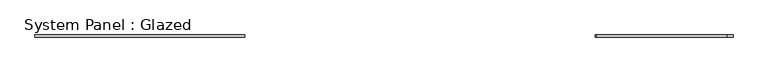
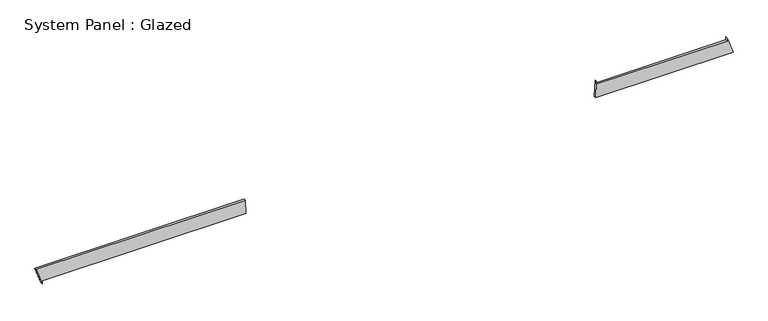
"""IFC4 building model written with IfcOpenShell, lengths in millimetres: plate geometry, System Panel : Glazed."""

from ifc_helpers import new_model, si_unit, frame, origin, place, context, project, spatial, polyline, outline, extrude, source, transform, mapped, element, save


def system_panel_glazed_a00b4466(model_context):
    return source(origin(), model_context, "Body", "SweptSolid", [
        extrude(outline(polyline([(0.0, -3957.6016429), (35.3553391, -3957.6016429), (35.3553391, -1604.6616071), (199.1260346, -1608.2248141), (199.0835123, -4027.0288897), (0.0, -3957.6016429)])), frame((0.0, -49.5, 0.0), z_axis=(0.0, 1.0, 0.0), x_axis=(0.0, 0.0, 1.0)), (0.0, 0.0, 1.0), 25.0),
        extrude(outline(polyline([(35.3553391, 2439.6918157), (35.3553391, 4027.0288897), (234.5792262, 3957.9376669), (199.2238871, 3957.9382884), (199.1973137, 2446.3571293), (234.5526528, 2446.3565077), (35.3553391, 2439.6918157)])), frame((0.0, -49.5, 0.0), z_axis=(0.0, 1.0, 0.0), x_axis=(0.0, 0.0, 1.0)), (0.0, 0.0, 1.0), 25.0),
    ])


if __name__ == "__main__":
    model = new_model("IFC4")
    model_context = context("Model", 3, world=origin())
    ifc_project = project(units=[si_unit("LENGTHUNIT", "METRE", prefix="MILLI")], contexts=[model_context])
    site = spatial("IfcSite", under=ifc_project)
    building = spatial("IfcBuilding", under=site)
    placement = place(None, origin())
    system_panel_glazed_shape = system_panel_glazed_a00b4466(model_context)
    element("IfcPlate", 1, ObjectType="System Panel : Glazed", at=placement, inside=building, context=model_context, shape_type="MappedRepresentation", body=[
        mapped(system_panel_glazed_shape, transform((0.0, 0.0, 0.0), x_axis=(1.0, 0.0, 0.0), y_axis=(0.0, 1.0, 0.0), z_axis=(0.0, 0.0, 1.0))),
    ])
    save(model, "model.ifc")

# Revit data of these elements
# Element 1 (IfcPlate, "System Panel : Glazed")
#   Materials on its faces: "Glass"
# Materials
#   "Glass": class "Glass", colour RGB 218 227 224, transparency 0.85, Description = "Soda Lime Glass", Cost = 0
